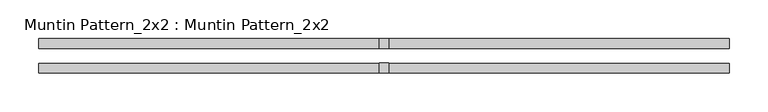
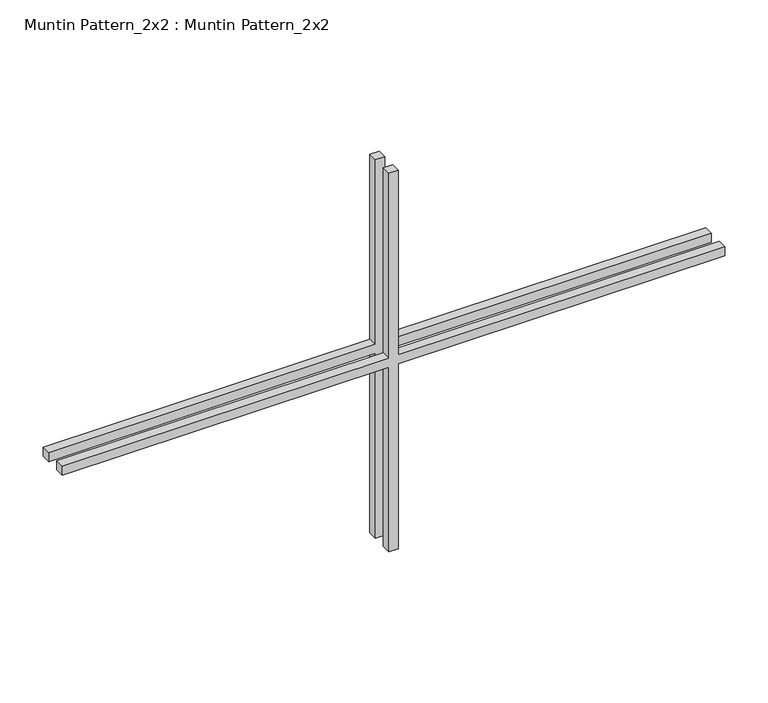
"""IFC4 building model written with IfcOpenShell, lengths in millimetres: proxy geometry, Muntin Pattern_2x2 : Muntin Pattern_2x2."""

from ifc_helpers import new_model, si_unit, frame, origin, place, context, project, spatial, polyline, outline, extrude, source, transform, mapped, element, save


def muntin_pattern_2x2_muntin_pattern_2x2_e5078fa2(model_context):
    return source(origin(), model_context, "Body", "SweptSolid", [
        extrude(outline(polyline([(274.6375, -6.35), (274.6375, -444.5), (261.9375, -444.5), (261.9375, -6.35), (0.0, -6.35), (0.0, 6.35), (261.9375, 6.35), (261.9375, 444.5), (274.6375, 444.5), (274.6375, 6.35), (536.575, 6.35), (536.575, -6.35), (274.6375, -6.35)])), frame((0.0, 9.525, 0.0), z_axis=(0.0, 1.0, 0.0), x_axis=(0.0, 0.0, 1.0)), (0.0, 0.0, 1.0), 12.7),
        extrude(outline(polyline([(274.6375, -6.35), (274.6375, -444.5), (261.9375, -444.5), (261.9375, -6.35), (0.0, -6.35), (0.0, 6.35), (261.9375, 6.35), (261.9375, 444.5), (274.6375, 444.5), (274.6375, 6.35), (536.575, 6.35), (536.575, -6.35), (274.6375, -6.35)])), frame((0.0, -22.225, 0.0), z_axis=(0.0, 1.0, 0.0), x_axis=(0.0, 0.0, 1.0)), (0.0, 0.0, 1.0), 12.7),
    ])


if __name__ == "__main__":
    model = new_model("IFC4")
    model_context = context("Model", 3, world=origin())
    ifc_project = project(units=[si_unit("LENGTHUNIT", "METRE", prefix="MILLI")], contexts=[model_context])
    site = spatial("IfcSite", under=ifc_project)
    building = spatial("IfcBuilding", under=site)
    placement = place(None, origin())
    muntin_pattern_2x2_muntin_pattern_2x2_shape = muntin_pattern_2x2_muntin_pattern_2x2_e5078fa2(model_context)
    element("IfcBuildingElementProxy", 1, Name="Muntin Pattern_2x2 : Muntin Pattern_2x2", ObjectType="Muntin Pattern_2x2 : Muntin Pattern_2x2", at=placement, inside=building, context=model_context, shape_type="MappedRepresentation", body=[
        mapped(muntin_pattern_2x2_muntin_pattern_2x2_shape, transform((0.0, 0.0, 0.0), x_axis=(1.0, 0.0, 0.0), y_axis=(0.0, 1.0, 0.0), z_axis=(0.0, 0.0, 1.0))),
    ])
    save(model, "model.ifc")

# Revit data of these elements
# Type "Muntin Pattern_2x2 : Muntin Pattern_2x2"
#   Width [instance default] = 4' - 0"
#   Thickness = 0' - 0 1/2"
#   Height [instance default] = 4' - 0"
#   Distance = 0' - 0 3/4"
#   Interior Material [instance default] = none
#   Exterior Material [instance default] = none
# Element 1 (IfcBuildingElementProxy, "Muntin Pattern_2x2 : Muntin Pattern_2x2")
#   Width = 2' - 11"
#   Height = 1' - 9 1/8"
#   Interior Material = Wood - Stained
#   Exterior Material = Clad - White
#   Materials on its faces: "Clad - White", "Wood - Stained"
# Materials
#   "Clad - White": class "Wood", colour RGB 242 242 238, transparency 0, Cost = 0
#   "Wood - Stained": class "Wood", colour RGB 224 178 126, transparency 0, Cost = 0
